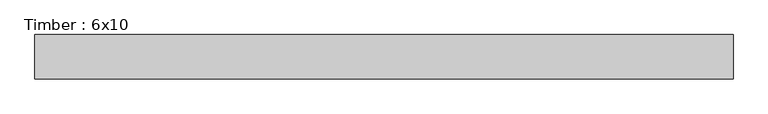
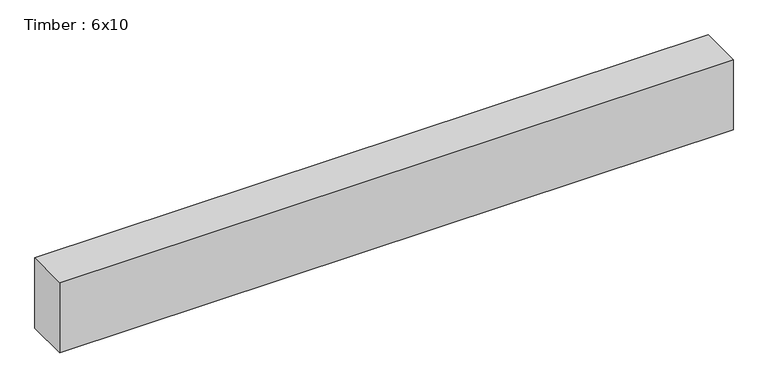
"""IFC4 building model written with IfcOpenShell, lengths in millimetres: beam geometry, Timber : 6x10."""

import ifcopenshell
import ifcopenshell.guid

model = None  # the IFC model being written
_history = None  # IfcOwnerHistory: only IFC2X3 demands one
_inside = {}  # id of a spatial element -> (the spatial element, [elements in it])
_under = {}  # id of a project, library or spatial element -> (it, [spatial elements below it])
_declared = {}  # id of a project -> (the project, [libraries it declares])
_typed = {}  # id of a type object -> (the type object, [elements of that type])
_made_of = {}  # id of a material, layer set ... -> (it, [elements and type objects made of it])


def new_model(schema):
    """Start an empty IFC model of exactly this schema.

    Asked for "IFC4X3", IfcOpenShell would pick the latest addendum, in which some entities
    have other attributes; the version numbers below select the first issue.
    IFC2X3 requires an IfcOwnerHistory on every rooted entity: one is made here for all.
    """
    global model, _history
    if schema == "IFC4X3":
        model = ifcopenshell.file(schema_version=(4, 3, 0, 0))
    else:
        model = ifcopenshell.file(schema=schema)
    _inside.clear()
    _under.clear()
    _declared.clear()
    _typed.clear()
    _made_of.clear()
    _history = None
    if model.schema == "IFC2X3":
        org = make("IfcOrganization", Name="unknown")
        user = make(
            "IfcPersonAndOrganization",
            ThePerson=make("IfcPerson", FamilyName="unknown"),
            TheOrganization=org,
        )
        app = make(
            "IfcApplication",
            ApplicationDeveloper=org,
            Version="unknown",
            ApplicationFullName="unknown",
            ApplicationIdentifier="unknown",
        )
        _history = make(
            "IfcOwnerHistory",
            OwningUser=user,
            OwningApplication=app,
            ChangeAction="ADDED",
            CreationDate=0,
        )
    return model


def make(cls, **values):
    """One entity of the class cls with the attributes given. An attribute that is None is left unset."""
    return model.create_entity(
        cls, **{name: value for name, value in values.items() if value is not None}
    )


def rooted(cls, **values):
    """An entity with a GlobalId (a new one), such as an element, a storey or a relation."""
    return make(cls, GlobalId=ifcopenshell.guid.new(), OwnerHistory=_history, **values)


def si_unit(unit_type, name, prefix=None):
    """IfcSIUnit, for example si_unit("LENGTHUNIT", "METRE", prefix="MILLI")."""
    return make("IfcSIUnit", UnitType=unit_type, Prefix=prefix, Name=name)


def assignment(units):
    """IfcUnitAssignment: the units of a project."""
    return None if units is None else make("IfcUnitAssignment", Units=units)


def point(xyz):
    """IfcCartesianPoint."""
    return None if xyz is None else make("IfcCartesianPoint", Coordinates=xyz)


def direction(xyz):
    """IfcDirection."""
    return None if xyz is None else make("IfcDirection", DirectionRatios=xyz)


def frame(location, z_axis=None, x_axis=None):
    """IfcAxis2Placement3D, a coordinate frame: its origin and axes. An axis left out is left unset."""
    return make(
        "IfcAxis2Placement3D",
        Location=point(location),
        Axis=direction(z_axis),
        RefDirection=direction(x_axis),
    )


def origin():
    """The frame at (0, 0, 0) with its axes left unset."""
    return frame((0.0, 0.0, 0.0))


def place(relative_to, where):
    """IfcLocalPlacement: puts the frame where relative to a parent placement (None: the world)."""
    return make(
        "IfcLocalPlacement", PlacementRelTo=relative_to, RelativePlacement=where
    )


def context(
    kind, dimensions, precision=None, world=None, true_north=None, identifier=None
):
    """IfcGeometricRepresentationContext, for example the 3D "Model" context."""
    return make(
        "IfcGeometricRepresentationContext",
        ContextIdentifier=identifier,
        ContextType=kind,
        CoordinateSpaceDimension=dimensions,
        Precision=precision,
        WorldCoordinateSystem=world,
        TrueNorth=true_north,
    )


def project(units=None, contexts=None):
    """IfcProject with its units and contexts."""
    return rooted(
        "IfcProject",
        Name="project",
        RepresentationContexts=contexts,
        UnitsInContext=assignment(units),
    )


def spatial(cls, under=None, at=None, **own):
    """A site, building, storey or space (cls), placed at a placement, below another one or the project."""
    s = rooted(cls, ObjectPlacement=at, **own)
    if under is not None:
        _under.setdefault(under.id(), (under, []))[1].append(s)
    return s


def polyline(points):
    """IfcPolyline through the points."""
    return make("IfcPolyline", Points=[point(p) for p in points])


def outline(outer, holes=None, kind="AREA"):
    """IfcArbitraryClosedProfileDef: a profile drawn as a closed curve; with holes, ...WithVoids."""
    if holes is None:
        return make("IfcArbitraryClosedProfileDef", ProfileType=kind, OuterCurve=outer)
    return make(
        "IfcArbitraryProfileDefWithVoids",
        ProfileType=kind,
        OuterCurve=outer,
        InnerCurves=holes,
    )


def extrude(swept, where, along, depth):
    """IfcExtrudedAreaSolid: the profile swept, set in the frame where, extruded along a direction by depth."""
    return make(
        "IfcExtrudedAreaSolid",
        SweptArea=swept,
        Position=where,
        ExtrudedDirection=direction(along),
        Depth=depth,
    )


def shape(context_of_items, identifier, shape_type, items):
    """IfcShapeRepresentation: the items that make up one representation, for example the "Body"."""
    return make(
        "IfcShapeRepresentation",
        ContextOfItems=context_of_items,
        RepresentationIdentifier=identifier,
        RepresentationType=shape_type,
        Items=items,
    )


def source(mapping_origin, context_of_items, identifier, shape_type, items):
    """IfcRepresentationMap: a shape defined once, which mapped items show again and again."""
    return make(
        "IfcRepresentationMap",
        MappingOrigin=mapping_origin,
        MappedRepresentation=shape(context_of_items, identifier, shape_type, items),
    )


def transform(
    local_origin,
    x_axis=None,
    y_axis=None,
    z_axis=None,
    scale=None,
    scale2=None,
    scale3=None,
    uniform=True,
):
    """IfcCartesianTransformationOperator3D, or its non-uniform kind. x_axis, y_axis, z_axis: its Axis1, 2, 3."""
    if uniform:
        return make(
            "IfcCartesianTransformationOperator3D",
            Axis1=direction(x_axis),
            Axis2=direction(y_axis),
            LocalOrigin=point(local_origin),
            Scale=scale,
            Axis3=direction(z_axis),
        )
    return make(
        "IfcCartesianTransformationOperator3DnonUniform",
        Axis1=direction(x_axis),
        Axis2=direction(y_axis),
        LocalOrigin=point(local_origin),
        Scale=scale,
        Axis3=direction(z_axis),
        Scale2=scale2,
        Scale3=scale3,
    )


def mapped(mapping_source, mapping_target):
    """IfcMappedItem: shows the shape of a source again, moved by a transform."""
    return make(
        "IfcMappedItem", MappingSource=mapping_source, MappingTarget=mapping_target
    )


def made_of(thing, what):
    """Note that an element or type object is made of a material, layer set ...; save() writes the relation."""
    if what is not None:
        _made_of.setdefault(what.id(), (what, []))[1].append(thing)
    return thing


def element(
    cls,
    number,
    at=None,
    inside=None,
    cuts=None,
    type_object=None,
    material=None,
    context=None,
    identifier="Body",
    shape_type=None,
    held_by="IfcProductDefinitionShape",
    body=None,
    shapes=None,
    **own,
):
    """One element of the class cls, such as IfcWall. Its Tag is "e" and its number.

    at: its placement. inside: the storey or other place that contains it. cuts: it is an
    opening in that element (IfcRelVoidsElement). A single representation is given by context,
    identifier, shape_type and body (its items); several are given by shapes. held_by: the class
    of the entity that holds the representations. save() writes the other relations.
    """
    e = rooted(cls, Tag="e%d" % number, ObjectPlacement=at, **own)
    if body is not None:
        shapes = [shape(context, identifier, shape_type, body)]
    if shapes is not None:
        e.Representation = make(held_by, Representations=shapes)
    if inside is not None:
        _inside.setdefault(inside.id(), (inside, []))[1].append(e)
    if cuts is not None:
        rooted(
            "IfcRelVoidsElement", RelatingBuildingElement=cuts, RelatedOpeningElement=e
        )
    if type_object is not None:
        _typed.setdefault(type_object.id(), (type_object, []))[1].append(e)
    return made_of(e, material)


def aggregate(whole, parts):
    """IfcRelAggregates: a whole, such as a stair, and the parts it consists of."""
    return rooted("IfcRelAggregates", RelatingObject=whole, RelatedObjects=parts)


def save(model, path):
    """Write the relations noted so far, then the file.

    IfcRelAggregates (storeys below a building ...), IfcRelContainedInSpatialStructure (elements
    in a storey), IfcRelDefinesByType, IfcRelAssociatesMaterial and IfcRelDeclares: one each for
    every whole, place, type object, material and project.
    """
    for whole, parts in _under.values():
        aggregate(whole, parts)
    for where, things in _inside.values():
        rooted(
            "IfcRelContainedInSpatialStructure",
            RelatedElements=things,
            RelatingStructure=where,
        )
    for kind, things in _typed.values():
        rooted("IfcRelDefinesByType", RelatedObjects=things, RelatingType=kind)
    for what, things in _made_of.values():
        rooted("IfcRelAssociatesMaterial", RelatedObjects=things, RelatingMaterial=what)
    for by, libraries in _declared.values():
        rooted("IfcRelDeclares", RelatingContext=by, RelatedDefinitions=libraries)
    model.write(path)


def timber_6x10_97aa413e(model_context):
    return source(origin(), model_context, "Body", "SweptSolid", [
        extrude(outline(polyline([(1096.3279, 69.85), (1096.3279, -69.85), (-1091.5816749, -69.85), (-1091.5816749, 69.85), (1096.3279, 69.85)])), frame((0.0, 0.0, -120.65), z_axis=(0.0, 0.0, 1.0), x_axis=(1.0, 0.0, 0.0)), (0.0, 0.0, 1.0), 241.3),
    ])


if __name__ == "__main__":
    model = new_model("IFC4")
    model_context = context("Model", 3, world=origin())
    ifc_project = project(units=[si_unit("LENGTHUNIT", "METRE", prefix="MILLI")], contexts=[model_context])
    site = spatial("IfcSite", under=ifc_project)
    building = spatial("IfcBuilding", under=site)
    placement = place(None, origin())
    timber_6x10_shape = timber_6x10_97aa413e(model_context)
    element("IfcBeam", 1, ObjectType="Timber : 6x10", at=placement, inside=building, context=model_context, shape_type="MappedRepresentation", body=[
        mapped(timber_6x10_shape, transform((0.0, 0.0, 0.0), x_axis=(1.0, 0.0, 0.0), y_axis=(0.0, 1.0, 0.0), z_axis=(0.0, 0.0, 1.0))),
    ])
    save(model, "model.ifc")

# Revit data of these elements
# Type "Timber : 6x10"
#   Assembly Code = "B10"
#   A = 0.362847 SF
#   Length [instance default] = 5' - 0"
#   b = 0' - 5 1/2"
#   d = 0' - 9 1/2"
#   Structural Material [instance default] = Softwood, Lumber
# Element 1 (IfcBeam, "Timber : 6x10")
#   Materials on its faces: "Softwood, Lumber"
# Materials
#   "Softwood, Lumber": class "Wood", colour RGB 144 113 62, transparency 0, Description = "Pinus Echinata", Cost = 0
